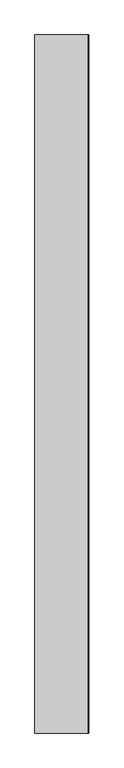
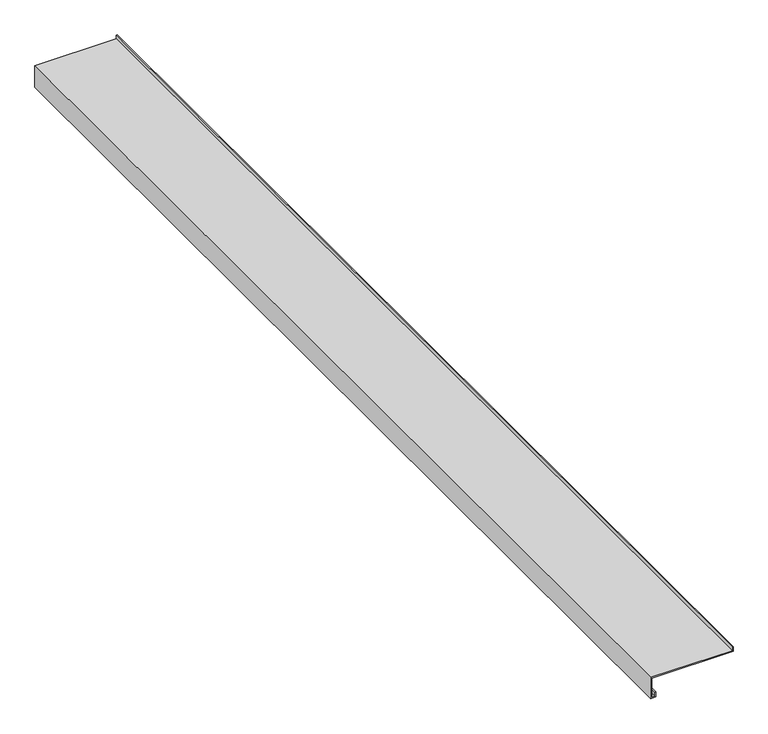
"""IFC4 building model written with IfcOpenShell, lengths in millimetres: proxy geometry, Flashing14:Flashing026:295295 : Flashing14:Flashing026:295295."""

from ifc_helpers import new_model, si_unit, frame, origin, place, context, project, spatial, polyline, outline, extrude, source, transform, mapped, element, save


def generic_models_d253baa9(model_context):
    return source(origin(), model_context, "Body", "SweptSolid", [
        extrude(outline(polyline([(36566.1804687, 2781.0440201), (36566.1804687, 2779.0440201), (36558.9851563, 2779.0440201), (36558.9851563, 2626.2595963), (36516.8054688, 2626.2595963), (36516.8054688, 2636.3194107), (36527.3601562, 2636.3194107), (36527.3601562, 2634.3194107), (36518.8054687, 2634.3194107), (36518.8054687, 2628.2595963), (36556.9851562, 2628.2595963), (36556.9851562, 2781.0440201), (36566.1804687, 2781.0440201)])), frame((0.0, 1276.4895464, 0.0), z_axis=(0.0, 1.0, 0.0), x_axis=(0.0, 0.0, 1.0)), (0.0, 0.0, 1.0), 2000.0),
    ])


if __name__ == "__main__":
    model = new_model("IFC4")
    model_context = context("Model", 3, world=origin())
    ifc_project = project(units=[si_unit("LENGTHUNIT", "METRE", prefix="MILLI")], contexts=[model_context])
    site = spatial("IfcSite", under=ifc_project)
    building = spatial("IfcBuilding", under=site)
    placement = place(None, origin())
    generic_models_shape = generic_models_d253baa9(model_context)
    element("IfcBuildingElementProxy", 1, Name="Flashing14:Flashing026:295295 : Flashing14:Flashing026:295295", ObjectType="Flashing14:Flashing026:295295 : Flashing14:Flashing026:295295", at=placement, inside=building, context=model_context, shape_type="MappedRepresentation", body=[
        mapped(generic_models_shape, transform((0.0, 0.0, 0.0), x_axis=(1.0, 0.0, 0.0), y_axis=(0.0, 1.0, 0.0), z_axis=(0.0, 0.0, 1.0))),
    ])
    save(model, "model.ifc")

# Revit data of these elements
# Type "Flashing14:Flashing026:295295 : Flashing14:Flashing026:295295"
#   NameOverride = "Flashing14:Flashing026:295295"
#   ObjectTypeOverride = "Flashing14:Flashing026"
#   Reference = "Flashing026"
#   Category = "Generic Models"
#   Tag = "295295"
# Element 1 (IfcBuildingElementProxy, "Flashing14:Flashing026:295295 : Flashing14:Flashing026:295295")
#   Materials on its faces: "COPPER SILL PAN AT ALL EXTERIOR WINDOWS/DOORS PER DETAIL 1/A4.1"
# Materials
#   "COPPER SILL PAN AT ALL EXTERIOR WINDOWS/DOORS PER DETAIL 1/A4.1": class "Unassigned", colour RGB 255 170 255, transparency 0, Cost = 0
